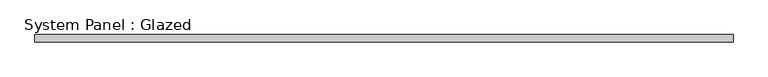
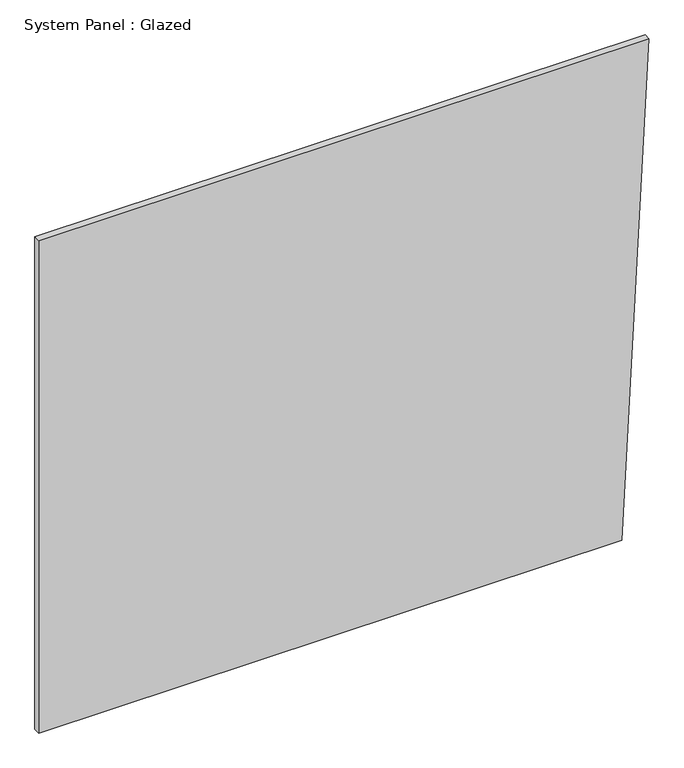
"""IFC4 building model written with IfcOpenShell, lengths in millimetres: plate geometry, System Panel : Glazed."""

from ifc_helpers import new_model, si_unit, frame, origin, place, context, project, spatial, polyline, outline, extrude, source, transform, mapped, element, save


def system_panel_glazed_7a24276e(model_context):
    return source(origin(), model_context, "Body", "SweptSolid", [
        extrude(outline(polyline([(0.0, -1222.0297486), (0.0, 1112.8894655), (2085.3785982, 1222.0297486), (2085.3785982, -1222.0297486), (0.0, -1222.0297486)])), frame((0.0, -44.45, 0.0), z_axis=(0.0, 1.0, 0.0), x_axis=(0.0, 0.0, 1.0)), (0.0, 0.0, 1.0), 25.4),
    ])


if __name__ == "__main__":
    model = new_model("IFC4")
    model_context = context("Model", 3, world=origin())
    ifc_project = project(units=[si_unit("LENGTHUNIT", "METRE", prefix="MILLI")], contexts=[model_context])
    site = spatial("IfcSite", under=ifc_project)
    building = spatial("IfcBuilding", under=site)
    placement = place(None, origin())
    system_panel_glazed_shape = system_panel_glazed_7a24276e(model_context)
    element("IfcPlate", 1, ObjectType="System Panel : Glazed", at=placement, inside=building, context=model_context, shape_type="MappedRepresentation", body=[
        mapped(system_panel_glazed_shape, transform((0.0, 0.0, 0.0), x_axis=(1.0, 0.0, 0.0), y_axis=(0.0, 1.0, 0.0), z_axis=(0.0, 0.0, 1.0))),
    ])
    save(model, "model.ifc")

# Revit data of these elements
# Type "System Panel : Glazed"
#   Construction Type Id = "GSP4R"
#   Analytic Construction = "1/8 in Pilkington single glazing"
#   Visual Light Transmittance = 0.9
#   Solar Heat Gain Coefficient = 0.86
#   Heat Transfer Coefficient (U) = 1.18115 BTU/(h·ft²·°F)
#   Define Thermal Properties by = 1
# Element 1 (IfcPlate, "System Panel : Glazed")
#   Materials on its faces: "Glass"
# Materials
#   "Glass": class "Glass", colour RGB 0 128 192, transparency 0.75, Description = "Soda Lime Glass", Cost = 0
